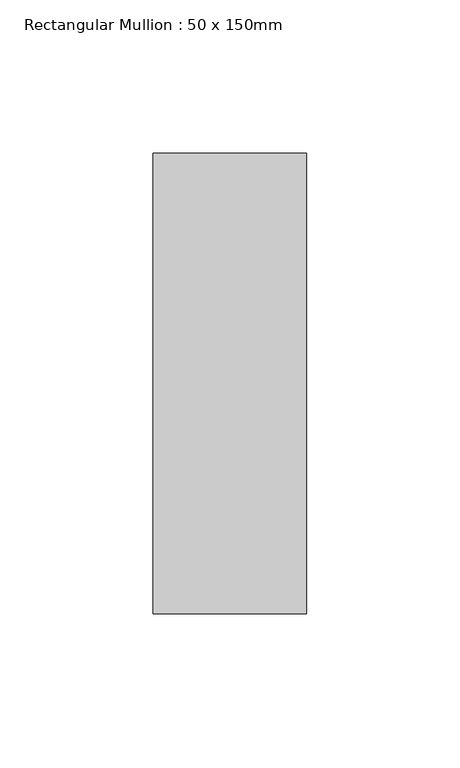
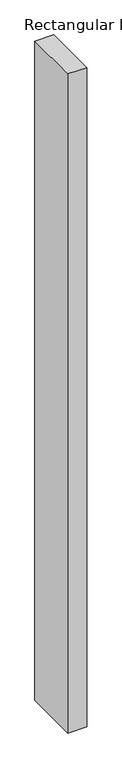
"""IFC4 building model written with IfcOpenShell, lengths in millimetres: member geometry, Rectangular Mullion : 50 x 150mm."""

from ifc_helpers import new_model, si_unit, frame, origin, place, context, project, spatial, polyline, outline, extrude, source, transform, mapped, element, save


def rectangular_mullion_50_x_150mm_82ddb8e0(model_context):
    return source(origin(), model_context, "Body", "SweptSolid", [
        extrude(outline(polyline([(25.0, 75.0), (25.0, -75.0), (-25.0, -75.0), (-25.0, 75.0), (25.0, 75.0)])), frame((0.0, 0.0, -1836.1666666), z_axis=(0.0, 0.0, 1.0), x_axis=(1.0, 0.0, 0.0)), (0.0, 0.0, 1.0), 1836.1666666),
    ])


if __name__ == "__main__":
    model = new_model("IFC4")
    model_context = context("Model", 3, world=origin())
    ifc_project = project(units=[si_unit("LENGTHUNIT", "METRE", prefix="MILLI")], contexts=[model_context])
    site = spatial("IfcSite", under=ifc_project)
    building = spatial("IfcBuilding", under=site)
    placement = place(None, origin())
    rectangular_mullion_50_x_150mm_shape = rectangular_mullion_50_x_150mm_82ddb8e0(model_context)
    element("IfcMember", 1, ObjectType="Rectangular Mullion : 50 x 150mm", at=placement, inside=building, context=model_context, shape_type="MappedRepresentation", body=[
        mapped(rectangular_mullion_50_x_150mm_shape, transform((0.0, 0.0, 0.0), x_axis=(1.0, 0.0, 0.0), y_axis=(0.0, 1.0, 0.0), z_axis=(0.0, 0.0, 1.0))),
    ])
    save(model, "model.ifc")

# Revit data of these elements
# Type "Rectangular Mullion : 50 x 150mm"
#   built-in parameter 1007304 = 0.492126 (stored number, unit not read)
#   built-in parameter 1007301 = 0.082021 (stored number, unit not read)
#   built-in parameter 1007300 = 0.082021 (stored number, unit not read)
# Element 1 (IfcMember, "Rectangular Mullion : 50 x 150mm")
#   Materials on its faces: "Metal - Aluminium"
# Materials
#   "Metal - Aluminium": class "Metal", colour RGB 247 247 247, transparency 0
